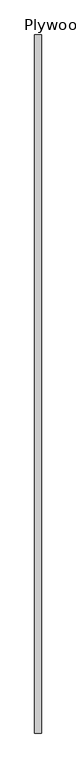
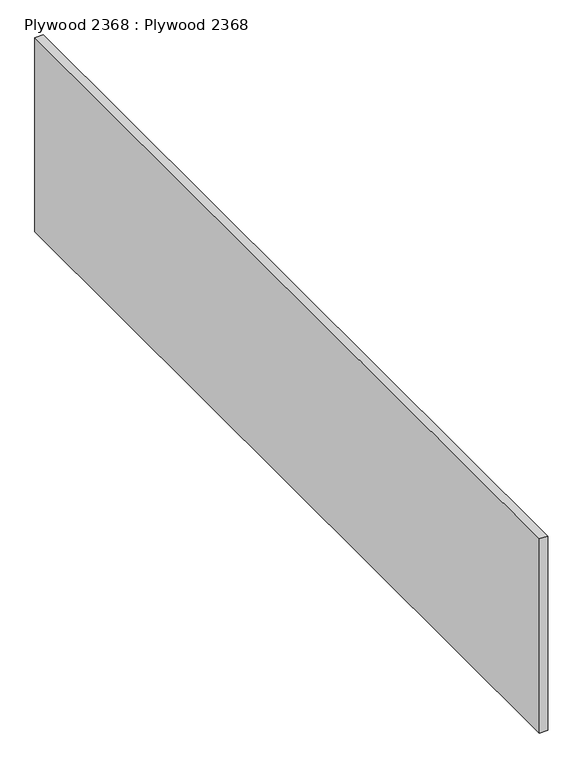
"""IFC4 building model written with IfcOpenShell, lengths in millimetres: proxy geometry, Plywood 2368 : Plywood 2368."""

from ifc_helpers import new_model, si_unit, frame, origin, place, context, project, spatial, polyline, outline, extrude, source, transform, mapped, element, save


def plywood_2368_plywood_2368_57cb3a2c(model_context):
    return source(origin(), model_context, "Body", "SweptSolid", [
        extrude(outline(polyline([(-4975.7038825, -1052.8906574), (-4994.7538825, -1052.8906574), (-4994.7538825, 947.1093426), (-4975.7038825, 947.1093426), (-4975.7038825, -1052.8906574)])), frame((0.0, 0.0, 39579.2960083), z_axis=(0.0, 0.0, 1.0), x_axis=(1.0, 0.0, 0.0)), (0.0, 0.0, 1.0), 469.8999917),
    ])


if __name__ == "__main__":
    model = new_model("IFC4")
    model_context = context("Model", 3, world=origin())
    ifc_project = project(units=[si_unit("LENGTHUNIT", "METRE", prefix="MILLI")], contexts=[model_context])
    site = spatial("IfcSite", under=ifc_project)
    building = spatial("IfcBuilding", under=site)
    placement = place(None, origin())
    plywood_2368_plywood_2368_shape = plywood_2368_plywood_2368_57cb3a2c(model_context)
    element("IfcBuildingElementProxy", 1, Name="Plywood 2368 : Plywood 2368", ObjectType="Plywood 2368 : Plywood 2368", at=placement, inside=building, context=model_context, shape_type="MappedRepresentation", body=[
        mapped(plywood_2368_plywood_2368_shape, transform((0.0, 0.0, 0.0), x_axis=(1.0, 0.0, 0.0), y_axis=(0.0, 1.0, 0.0), z_axis=(0.0, 0.0, 1.0))),
    ])
    save(model, "model.ifc")

# Revit data of these elements
# Type "Plywood 2368 : Plywood 2368"
#   NameOverride = "Plywood"
# Element 1 (IfcBuildingElementProxy, "Plywood 2368 : Plywood 2368")
#   Materials on its faces: "CDX PLYWOOD -  SEE STRUCTURAL DWGS"
# Materials
#   "CDX PLYWOOD -  SEE STRUCTURAL DWGS": class "Unassigned", colour RGB 177 130 114, transparency 0, Cost = 0
